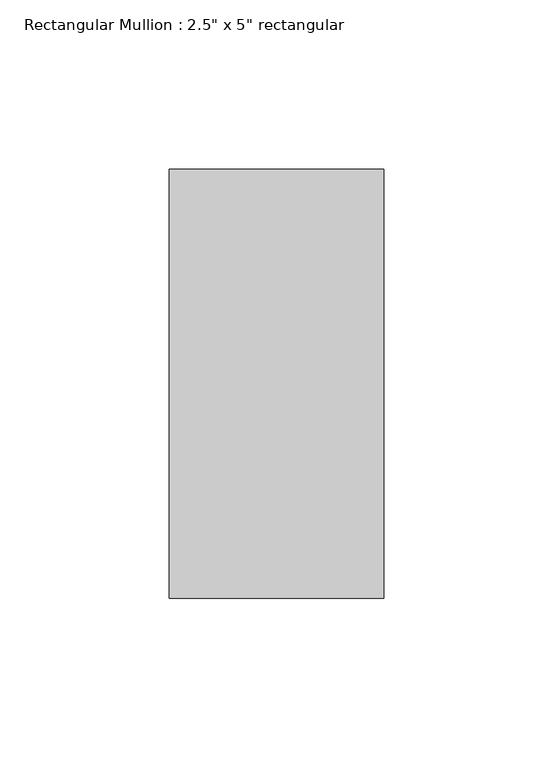
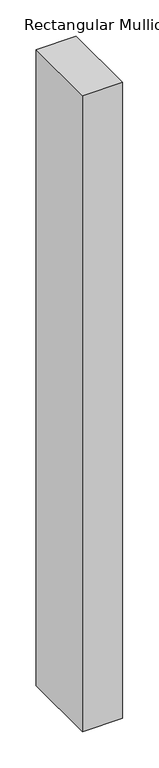
"""IFC4 building model written with IfcOpenShell, lengths in millimetres: member geometry."""

import ifcopenshell
import ifcopenshell.guid

model = None  # the IFC model being written
_history = None  # IfcOwnerHistory: only IFC2X3 demands one
_inside = {}  # id of a spatial element -> (the spatial element, [elements in it])
_under = {}  # id of a project, library or spatial element -> (it, [spatial elements below it])
_declared = {}  # id of a project -> (the project, [libraries it declares])
_typed = {}  # id of a type object -> (the type object, [elements of that type])
_made_of = {}  # id of a material, layer set ... -> (it, [elements and type objects made of it])


def new_model(schema):
    """Start an empty IFC model of exactly this schema.

    Asked for "IFC4X3", IfcOpenShell would pick the latest addendum, in which some entities
    have other attributes; the version numbers below select the first issue.
    IFC2X3 requires an IfcOwnerHistory on every rooted entity: one is made here for all.
    """
    global model, _history
    if schema == "IFC4X3":
        model = ifcopenshell.file(schema_version=(4, 3, 0, 0))
    else:
        model = ifcopenshell.file(schema=schema)
    _inside.clear()
    _under.clear()
    _declared.clear()
    _typed.clear()
    _made_of.clear()
    _history = None
    if model.schema == "IFC2X3":
        org = make("IfcOrganization", Name="unknown")
        user = make(
            "IfcPersonAndOrganization",
            ThePerson=make("IfcPerson", FamilyName="unknown"),
            TheOrganization=org,
        )
        app = make(
            "IfcApplication",
            ApplicationDeveloper=org,
            Version="unknown",
            ApplicationFullName="unknown",
            ApplicationIdentifier="unknown",
        )
        _history = make(
            "IfcOwnerHistory",
            OwningUser=user,
            OwningApplication=app,
            ChangeAction="ADDED",
            CreationDate=0,
        )
    return model


def make(cls, **values):
    """One entity of the class cls with the attributes given. An attribute that is None is left unset."""
    return model.create_entity(
        cls, **{name: value for name, value in values.items() if value is not None}
    )


def rooted(cls, **values):
    """An entity with a GlobalId (a new one), such as an element, a storey or a relation."""
    return make(cls, GlobalId=ifcopenshell.guid.new(), OwnerHistory=_history, **values)


def si_unit(unit_type, name, prefix=None):
    """IfcSIUnit, for example si_unit("LENGTHUNIT", "METRE", prefix="MILLI")."""
    return make("IfcSIUnit", UnitType=unit_type, Prefix=prefix, Name=name)


def assignment(units):
    """IfcUnitAssignment: the units of a project."""
    return None if units is None else make("IfcUnitAssignment", Units=units)


def point(xyz):
    """IfcCartesianPoint."""
    return None if xyz is None else make("IfcCartesianPoint", Coordinates=xyz)


def direction(xyz):
    """IfcDirection."""
    return None if xyz is None else make("IfcDirection", DirectionRatios=xyz)


def frame(location, z_axis=None, x_axis=None):
    """IfcAxis2Placement3D, a coordinate frame: its origin and axes. An axis left out is left unset."""
    return make(
        "IfcAxis2Placement3D",
        Location=point(location),
        Axis=direction(z_axis),
        RefDirection=direction(x_axis),
    )


def origin():
    """The frame at (0, 0, 0) with its axes left unset."""
    return frame((0.0, 0.0, 0.0))


def place(relative_to, where):
    """IfcLocalPlacement: puts the frame where relative to a parent placement (None: the world)."""
    return make(
        "IfcLocalPlacement", PlacementRelTo=relative_to, RelativePlacement=where
    )


def context(
    kind, dimensions, precision=None, world=None, true_north=None, identifier=None
):
    """IfcGeometricRepresentationContext, for example the 3D "Model" context."""
    return make(
        "IfcGeometricRepresentationContext",
        ContextIdentifier=identifier,
        ContextType=kind,
        CoordinateSpaceDimension=dimensions,
        Precision=precision,
        WorldCoordinateSystem=world,
        TrueNorth=true_north,
    )


def project(units=None, contexts=None):
    """IfcProject with its units and contexts."""
    return rooted(
        "IfcProject",
        Name="project",
        RepresentationContexts=contexts,
        UnitsInContext=assignment(units),
    )


def spatial(cls, under=None, at=None, **own):
    """A site, building, storey or space (cls), placed at a placement, below another one or the project."""
    s = rooted(cls, ObjectPlacement=at, **own)
    if under is not None:
        _under.setdefault(under.id(), (under, []))[1].append(s)
    return s


def polyline(points):
    """IfcPolyline through the points."""
    return make("IfcPolyline", Points=[point(p) for p in points])


def outline(outer, holes=None, kind="AREA"):
    """IfcArbitraryClosedProfileDef: a profile drawn as a closed curve; with holes, ...WithVoids."""
    if holes is None:
        return make("IfcArbitraryClosedProfileDef", ProfileType=kind, OuterCurve=outer)
    return make(
        "IfcArbitraryProfileDefWithVoids",
        ProfileType=kind,
        OuterCurve=outer,
        InnerCurves=holes,
    )


def extrude(swept, where, along, depth):
    """IfcExtrudedAreaSolid: the profile swept, set in the frame where, extruded along a direction by depth."""
    return make(
        "IfcExtrudedAreaSolid",
        SweptArea=swept,
        Position=where,
        ExtrudedDirection=direction(along),
        Depth=depth,
    )


def shape(context_of_items, identifier, shape_type, items):
    """IfcShapeRepresentation: the items that make up one representation, for example the "Body"."""
    return make(
        "IfcShapeRepresentation",
        ContextOfItems=context_of_items,
        RepresentationIdentifier=identifier,
        RepresentationType=shape_type,
        Items=items,
    )


def source(mapping_origin, context_of_items, identifier, shape_type, items):
    """IfcRepresentationMap: a shape defined once, which mapped items show again and again."""
    return make(
        "IfcRepresentationMap",
        MappingOrigin=mapping_origin,
        MappedRepresentation=shape(context_of_items, identifier, shape_type, items),
    )


def transform(
    local_origin,
    x_axis=None,
    y_axis=None,
    z_axis=None,
    scale=None,
    scale2=None,
    scale3=None,
    uniform=True,
):
    """IfcCartesianTransformationOperator3D, or its non-uniform kind. x_axis, y_axis, z_axis: its Axis1, 2, 3."""
    if uniform:
        return make(
            "IfcCartesianTransformationOperator3D",
            Axis1=direction(x_axis),
            Axis2=direction(y_axis),
            LocalOrigin=point(local_origin),
            Scale=scale,
            Axis3=direction(z_axis),
        )
    return make(
        "IfcCartesianTransformationOperator3DnonUniform",
        Axis1=direction(x_axis),
        Axis2=direction(y_axis),
        LocalOrigin=point(local_origin),
        Scale=scale,
        Axis3=direction(z_axis),
        Scale2=scale2,
        Scale3=scale3,
    )


def mapped(mapping_source, mapping_target):
    """IfcMappedItem: shows the shape of a source again, moved by a transform."""
    return make(
        "IfcMappedItem", MappingSource=mapping_source, MappingTarget=mapping_target
    )


def made_of(thing, what):
    """Note that an element or type object is made of a material, layer set ...; save() writes the relation."""
    if what is not None:
        _made_of.setdefault(what.id(), (what, []))[1].append(thing)
    return thing


def element(
    cls,
    number,
    at=None,
    inside=None,
    cuts=None,
    type_object=None,
    material=None,
    context=None,
    identifier="Body",
    shape_type=None,
    held_by="IfcProductDefinitionShape",
    body=None,
    shapes=None,
    **own,
):
    """One element of the class cls, such as IfcWall. Its Tag is "e" and its number.

    at: its placement. inside: the storey or other place that contains it. cuts: it is an
    opening in that element (IfcRelVoidsElement). A single representation is given by context,
    identifier, shape_type and body (its items); several are given by shapes. held_by: the class
    of the entity that holds the representations. save() writes the other relations.
    """
    e = rooted(cls, Tag="e%d" % number, ObjectPlacement=at, **own)
    if body is not None:
        shapes = [shape(context, identifier, shape_type, body)]
    if shapes is not None:
        e.Representation = make(held_by, Representations=shapes)
    if inside is not None:
        _inside.setdefault(inside.id(), (inside, []))[1].append(e)
    if cuts is not None:
        rooted(
            "IfcRelVoidsElement", RelatingBuildingElement=cuts, RelatedOpeningElement=e
        )
    if type_object is not None:
        _typed.setdefault(type_object.id(), (type_object, []))[1].append(e)
    return made_of(e, material)


def aggregate(whole, parts):
    """IfcRelAggregates: a whole, such as a stair, and the parts it consists of."""
    return rooted("IfcRelAggregates", RelatingObject=whole, RelatedObjects=parts)


def save(model, path):
    """Write the relations noted so far, then the file.

    IfcRelAggregates (storeys below a building ...), IfcRelContainedInSpatialStructure (elements
    in a storey), IfcRelDefinesByType, IfcRelAssociatesMaterial and IfcRelDeclares: one each for
    every whole, place, type object, material and project.
    """
    for whole, parts in _under.values():
        aggregate(whole, parts)
    for where, things in _inside.values():
        rooted(
            "IfcRelContainedInSpatialStructure",
            RelatedElements=things,
            RelatingStructure=where,
        )
    for kind, things in _typed.values():
        rooted("IfcRelDefinesByType", RelatedObjects=things, RelatingType=kind)
    for what, things in _made_of.values():
        rooted("IfcRelAssociatesMaterial", RelatedObjects=things, RelatingMaterial=what)
    for by, libraries in _declared.values():
        rooted("IfcRelDeclares", RelatingContext=by, RelatedDefinitions=libraries)
    model.write(path)


def member_a715cb85(model_context):
    return source(origin(), model_context, "Body", "SweptSolid", [
        extrude(outline(polyline([(31.75, 63.5), (31.75, -63.5), (-31.75, -63.5), (-31.75, 63.5), (31.75, 63.5)])), frame((0.0, 0.0, -1066.8), z_axis=(0.0, 0.0, 1.0), x_axis=(1.0, 0.0, 0.0)), (0.0, 0.0, 1.0), 1066.8),
    ])


if __name__ == "__main__":
    model = new_model("IFC4")
    model_context = context("Model", 3, world=origin())
    ifc_project = project(units=[si_unit("LENGTHUNIT", "METRE", prefix="MILLI")], contexts=[model_context])
    site = spatial("IfcSite", under=ifc_project)
    building = spatial("IfcBuilding", under=site)
    placement = place(None, origin())
    member_shape = member_a715cb85(model_context)
    element("IfcMember", 1, ObjectType="Rectangular Mullion : 2.5\" x 5\" rectangular", at=placement, inside=building, context=model_context, shape_type="MappedRepresentation", body=[
        mapped(member_shape, transform((0.0, 0.0, 0.0), x_axis=(1.0, 0.0, 0.0), y_axis=(0.0, 1.0, 0.0), z_axis=(0.0, 0.0, 1.0))),
    ])
    save(model, "model.ifc")

# Revit data of these elements
# Type "Rectangular Mullion : 2.5\" x 5\" rectangular"
#   built-in parameter 1007304 = 0.416667 (stored number, unit not read)
#   built-in parameter 1007301 = 0.104167 (stored number, unit not read)
#   built-in parameter 1007300 = 0.104167 (stored number, unit not read)
# Element 1 (IfcMember, "Rectangular Mullion : 2.5\" x 5\" rectangular")
#   Materials on its faces: "Metal - Aluminum"
# Materials
#   "Metal - Aluminum": class "Metal", colour RGB 140 140 140, transparency 0
